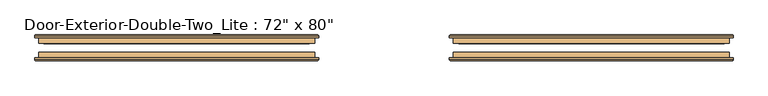
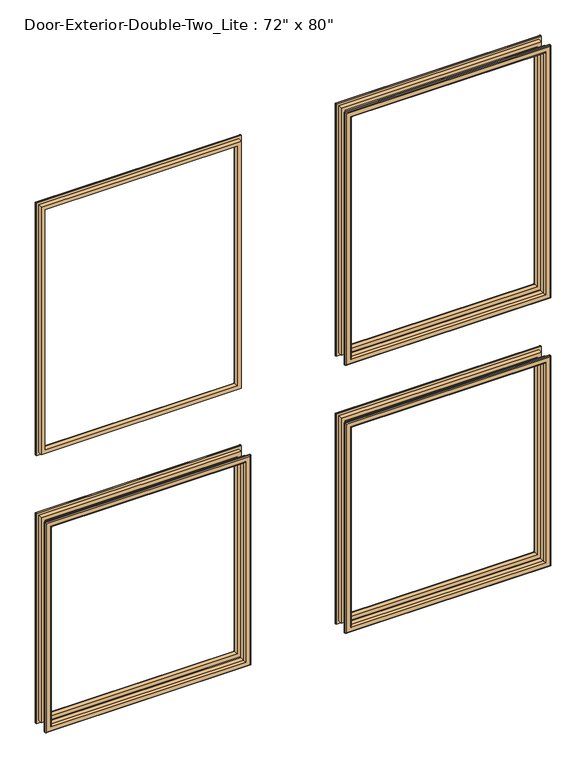
"""IFC4 building model written with IfcOpenShell, lengths in millimetres: door geometry."""

from ifc_helpers import new_model, si_unit, frame, origin, place, context, project, spatial, ellipse_curve, source, transform, mapped, element, save
from ifc_brep_helpers import plane_surface, cylinder_surface, advanced_brep


def door_4556e5f4(model_context):
    return source(origin(), model_context, "Body", "AdvancedBrep", [
        advanced_brep(
        [(-762.0, 66.675, 914.4), (-762.0, 79.375, 914.4), (-762.0, 79.375, 254.0), (-762.0, 66.675, 254.0), (-750.0, 80.375, 902.4), (-750.0, 66.675, 902.4), (-750.0, 66.675, 266.0), (-750.0, 80.375, 266.0), (-755.0, 85.375, 907.4), (-755.0, 85.375, 261.0), (-770.0, 83.375, 922.4), (-768.0, 85.375, 920.4), (-768.0, 85.375, 248.0), (-770.0, 83.375, 246.0), (-770.0, 79.375, 922.4), (-770.0, 79.375, 246.0), (-152.4, 79.375, 254.0), (-152.4, 66.675, 254.0), (-164.4, 66.675, 266.0), (-164.4, 80.375, 266.0), (-159.4, 85.375, 261.0), (-146.4, 85.375, 248.0), (-144.4, 83.375, 246.0), (-144.4, 79.375, 246.0), (-152.4, 79.375, 914.4), (-152.4, 66.675, 914.4), (-164.4, 66.675, 902.4), (-164.4, 80.375, 902.4), (-159.4, 85.375, 907.4), (-146.4, 85.375, 920.4), (-144.4, 83.375, 922.4), (-144.4, 79.375, 922.4)],
        [
            (0, 1),
            (1, 2),
            (2, 3),
            (3, 0),
            (4, 5),
            (5, 6),
            (6, 7),
            (7, 4),
            (8, 4, ellipse_curve(frame((-755.0, 80.375, 907.4), z_axis=(-0.7071067811865475, 0.0, -0.7071067811865475), x_axis=(-0.7071067811865474, 0.0, 0.7071067811865476)), 7.0710678, 5.0)),
            (7, 9, ellipse_curve(frame((-755.0, 80.375, 261.0), z_axis=(-0.7071067811865475, 0.0, 0.7071067811865475), x_axis=(0.7071067811865474, 0.0, 0.7071067811865476)), 7.0710678, 5.0)),
            (9, 8),
            (10, 11, ellipse_curve(frame((-768.0, 83.375, 920.4), z_axis=(-0.7071067811865475, 0.0, -0.7071067811865475), x_axis=(-0.7071067811865474, 0.0, 0.7071067811865476)), 2.8284271, 2.0)),
            (11, 12),
            (12, 13, ellipse_curve(frame((-768.0, 83.375, 248.0), z_axis=(-0.7071067811865475, 0.0, 0.7071067811865475), x_axis=(0.7071067811865474, 0.0, 0.7071067811865476)), 2.8284271, 2.0)),
            (13, 10),
            (14, 10),
            (13, 15),
            (15, 14),
            (2, 16),
            (16, 17),
            (17, 3),
            (6, 18),
            (18, 19),
            (19, 7),
            (19, 20, ellipse_curve(frame((-159.4, 80.375, 261.0), z_axis=(-0.7071067811865475, 0.0, -0.7071067811865475), x_axis=(-0.7071067811865476, 0.0, 0.7071067811865474)), 7.0710678, 5.0)),
            (20, 9),
            (12, 21),
            (21, 22, ellipse_curve(frame((-146.4, 83.375, 248.0), z_axis=(-0.7071067811865475, 0.0, -0.7071067811865475), x_axis=(-0.7071067811865476, 0.0, 0.7071067811865474)), 2.8284271, 2.0)),
            (22, 13),
            (22, 23),
            (23, 15),
            (16, 24),
            (24, 25),
            (25, 17),
            (18, 26),
            (26, 27),
            (27, 19),
            (27, 28, ellipse_curve(frame((-159.4, 80.375, 907.4), z_axis=(0.7071067811865475, 0.0, -0.7071067811865475), x_axis=(-0.7071067811865474, 0.0, -0.7071067811865476)), 7.0710678, 5.0)),
            (28, 20),
            (21, 29),
            (29, 30, ellipse_curve(frame((-146.4, 83.375, 920.4), z_axis=(0.7071067811865475, 0.0, -0.7071067811865475), x_axis=(-0.7071067811865474, 0.0, -0.7071067811865476)), 2.8284271, 2.0)),
            (30, 22),
            (30, 31),
            (31, 23),
            (31, 14),
            (1, 24),
            (0, 25),
            (5, 26),
            (4, 27),
            (8, 28),
            (11, 29),
            (10, 30),
        ],
        [
            plane_surface(frame((-762.0, 79.375, 914.4), z_axis=(-1.0, 0.0, 0.0), x_axis=(0.0, 0.0, -1.0))),
            plane_surface(frame((-750.0, 66.675, 902.4), z_axis=(1.0, 0.0, 0.0), x_axis=(0.0, 0.0, -1.0))),
            cylinder_surface(frame((-755.0, 80.375, 914.4), z_axis=(0.0, 0.0, 1.0), x_axis=(-1.0, 0.0, 0.0)), 5.0),
            cylinder_surface(frame((-768.0, 83.375, 914.4), z_axis=(0.0, 0.0, 1.0), x_axis=(-1.0, 0.0, 0.0)), 2.0),
            plane_surface(frame((-770.0, 83.375, 922.4), z_axis=(-1.0, 0.0, 0.0), x_axis=(0.0, 0.0, -1.0))),
            plane_surface(frame((-762.0, 79.375, 254.0), z_axis=(0.0, 0.0, -1.0), x_axis=(1.0, 0.0, 0.0))),
            plane_surface(frame((-750.0, 66.675, 266.0), z_axis=(0.0, 0.0, 1.0), x_axis=(1.0, 0.0, 0.0))),
            cylinder_surface(frame((-762.0, 80.375, 261.0), z_axis=(-1.0, 0.0, 0.0), x_axis=(0.0, 0.0, -1.0)), 5.0),
            cylinder_surface(frame((-762.0, 83.375, 248.0), z_axis=(-1.0, 0.0, 0.0), x_axis=(0.0, 0.0, -1.0)), 2.0),
            plane_surface(frame((-770.0, 83.375, 246.0), z_axis=(0.0, 0.0, -1.0), x_axis=(1.0, 0.0, 0.0))),
            plane_surface(frame((-152.4, 79.375, 254.0), z_axis=(1.0, 0.0, 0.0), x_axis=(0.0, 0.0, 1.0))),
            plane_surface(frame((-164.4, 66.675, 266.0), z_axis=(-1.0, 0.0, 0.0), x_axis=(0.0, 0.0, 1.0))),
            cylinder_surface(frame((-159.4, 80.375, 254.0), z_axis=(0.0, 0.0, -1.0), x_axis=(1.0, 0.0, 0.0)), 5.0),
            cylinder_surface(frame((-146.4, 83.375, 254.0), z_axis=(0.0, 0.0, -1.0), x_axis=(1.0, 0.0, 0.0)), 2.0),
            plane_surface(frame((-144.4, 83.375, 246.0), z_axis=(1.0, 0.0, 0.0), x_axis=(0.0, 0.0, 1.0))),
            plane_surface(frame((-144.4, 79.375, 922.4), z_axis=(0.0, -1.0, 0.0), x_axis=(-1.0, 0.0, 0.0))),
            plane_surface(frame((-152.4, 79.375, 914.4), z_axis=(0.0, 0.0, 1.0), x_axis=(-1.0, 0.0, 0.0))),
            plane_surface(frame((-152.4, 66.675, 914.4), z_axis=(0.0, -1.0, 0.0), x_axis=(-1.0, 0.0, 0.0))),
            plane_surface(frame((-164.4, 66.675, 902.4), z_axis=(0.0, 0.0, -1.0), x_axis=(-1.0, 0.0, 0.0))),
            cylinder_surface(frame((-152.4, 80.375, 907.4), z_axis=(1.0, 0.0, 0.0), x_axis=(0.0, 0.0, 1.0)), 5.0),
            plane_surface(frame((-159.4, 85.375, 907.4), z_axis=(0.0, 1.0, 0.0), x_axis=(-1.0, 0.0, 0.0))),
            cylinder_surface(frame((-152.4, 83.375, 920.4), z_axis=(1.0, 0.0, 0.0), x_axis=(0.0, 0.0, 1.0)), 2.0),
            plane_surface(frame((-144.4, 83.375, 922.4), z_axis=(0.0, 0.0, 1.0), x_axis=(-1.0, 0.0, 0.0))),
        ],
        [
            (0, [[1, 2, 3, 4]]),
            (1, [[5, 6, 7, 8]]),
            (2, [[9, -8, 10, 11]]),
            (3, [[12, 13, 14, 15]]),
            (4, [[16, -15, 17, 18]]),
            (5, [[-3, 19, 20, 21]]),
            (6, [[-7, 22, 23, 24]]),
            (7, [[-10, -24, 25, 26]]),
            (8, [[-14, 27, 28, 29]]),
            (9, [[-17, -29, 30, 31]]),
            (10, [[-20, 32, 33, 34]]),
            (11, [[-23, 35, 36, 37]]),
            (12, [[-25, -37, 38, 39]]),
            (13, [[-28, 40, 41, 42]]),
            (14, [[-30, -42, 43, 44]]),
            (15, [[-31, -44, 45, -18], [46, -32, -19, -2]]),
            (16, [[-33, -46, -1, 47]]),
            (17, [[-21, -34, -47, -4], [48, -35, -22, -6]]),
            (18, [[-36, -48, -5, 49]]),
            (19, [[-38, -49, -9, 50]]),
            (20, [[51, -40, -27, -13], [-26, -39, -50, -11]]),
            (21, [[-41, -51, -12, 52]]),
            (22, [[-43, -52, -16, -45]]),
        ],
    ),
        advanced_brep(
        [(152.4, 66.675, 914.4), (152.4, 79.375, 914.4), (152.4, 79.375, 254.0), (152.4, 66.675, 254.0), (164.4, 80.375, 902.4), (164.4, 66.675, 902.4), (164.4, 66.675, 266.0), (164.4, 80.375, 266.0), (159.4, 85.375, 907.4), (159.4, 85.375, 261.0), (144.4, 83.375, 922.4), (146.4, 85.375, 920.4), (146.4, 85.375, 248.0), (144.4, 83.375, 246.0), (144.4, 79.375, 922.4), (144.4, 79.375, 246.0), (762.0, 79.375, 254.0), (762.0, 66.675, 254.0), (750.0, 66.675, 266.0), (750.0, 80.375, 266.0), (755.0, 85.375, 261.0), (768.0, 85.375, 248.0), (770.0, 83.375, 246.0), (770.0, 79.375, 246.0), (762.0, 79.375, 914.4), (762.0, 66.675, 914.4), (750.0, 66.675, 902.4), (750.0, 80.375, 902.4), (755.0, 85.375, 907.4), (768.0, 85.375, 920.4), (770.0, 83.375, 922.4), (770.0, 79.375, 922.4)],
        [
            (0, 1),
            (1, 2),
            (2, 3),
            (3, 0),
            (4, 5),
            (5, 6),
            (6, 7),
            (7, 4),
            (8, 4, ellipse_curve(frame((159.4, 80.375, 907.4), z_axis=(-0.7071067811865475, 0.0, -0.7071067811865475), x_axis=(-0.7071067811865474, 0.0, 0.7071067811865476)), 7.0710678, 5.0)),
            (7, 9, ellipse_curve(frame((159.4, 80.375, 261.0), z_axis=(-0.7071067811865475, 0.0, 0.7071067811865475), x_axis=(0.7071067811865474, 0.0, 0.7071067811865476)), 7.0710678, 5.0)),
            (9, 8),
            (10, 11, ellipse_curve(frame((146.4, 83.375, 920.4), z_axis=(-0.7071067811865475, 0.0, -0.7071067811865475), x_axis=(-0.7071067811865474, 0.0, 0.7071067811865476)), 2.8284271, 2.0)),
            (11, 12),
            (12, 13, ellipse_curve(frame((146.4, 83.375, 248.0), z_axis=(-0.7071067811865475, 0.0, 0.7071067811865475), x_axis=(0.7071067811865474, 0.0, 0.7071067811865476)), 2.8284271, 2.0)),
            (13, 10),
            (14, 10),
            (13, 15),
            (15, 14),
            (2, 16),
            (16, 17),
            (17, 3),
            (6, 18),
            (18, 19),
            (19, 7),
            (19, 20, ellipse_curve(frame((755.0, 80.375, 261.0), z_axis=(-0.7071067811865475, 0.0, -0.7071067811865475), x_axis=(-0.7071067811865476, 0.0, 0.7071067811865474)), 7.0710678, 5.0)),
            (20, 9),
            (12, 21),
            (21, 22, ellipse_curve(frame((768.0, 83.375, 248.0), z_axis=(-0.7071067811865475, 0.0, -0.7071067811865475), x_axis=(-0.7071067811865476, 0.0, 0.7071067811865474)), 2.8284271, 2.0)),
            (22, 13),
            (22, 23),
            (23, 15),
            (16, 24),
            (24, 25),
            (25, 17),
            (18, 26),
            (26, 27),
            (27, 19),
            (27, 28, ellipse_curve(frame((755.0, 80.375, 907.4), z_axis=(0.7071067811865475, 0.0, -0.7071067811865475), x_axis=(-0.7071067811865474, 0.0, -0.7071067811865476)), 7.0710678, 5.0)),
            (28, 20),
            (21, 29),
            (29, 30, ellipse_curve(frame((768.0, 83.375, 920.4), z_axis=(0.7071067811865475, 0.0, -0.7071067811865475), x_axis=(-0.7071067811865474, 0.0, -0.7071067811865476)), 2.8284271, 2.0)),
            (30, 22),
            (30, 31),
            (31, 23),
            (31, 14),
            (1, 24),
            (0, 25),
            (5, 26),
            (4, 27),
            (8, 28),
            (11, 29),
            (10, 30),
        ],
        [
            plane_surface(frame((152.4, 79.375, 914.4), z_axis=(-1.0, 0.0, 0.0), x_axis=(0.0, 0.0, -1.0))),
            plane_surface(frame((164.4, 66.675, 902.4), z_axis=(1.0, 0.0, 0.0), x_axis=(0.0, 0.0, -1.0))),
            cylinder_surface(frame((159.4, 80.375, 914.4), z_axis=(0.0, 0.0, 1.0), x_axis=(-1.0, 0.0, 0.0)), 5.0),
            cylinder_surface(frame((146.4, 83.375, 914.4), z_axis=(0.0, 0.0, 1.0), x_axis=(-1.0, 0.0, 0.0)), 2.0),
            plane_surface(frame((144.4, 83.375, 922.4), z_axis=(-1.0, 0.0, 0.0), x_axis=(0.0, 0.0, -1.0))),
            plane_surface(frame((152.4, 79.375, 254.0), z_axis=(0.0, 0.0, -1.0), x_axis=(1.0, 0.0, 0.0))),
            plane_surface(frame((164.4, 66.675, 266.0), z_axis=(0.0, 0.0, 1.0), x_axis=(1.0, 0.0, 0.0))),
            cylinder_surface(frame((152.4, 80.375, 261.0), z_axis=(-1.0, 0.0, 0.0), x_axis=(0.0, 0.0, -1.0)), 5.0),
            cylinder_surface(frame((152.4, 83.375, 248.0), z_axis=(-1.0, 0.0, 0.0), x_axis=(0.0, 0.0, -1.0)), 2.0),
            plane_surface(frame((144.4, 83.375, 246.0), z_axis=(0.0, 0.0, -1.0), x_axis=(1.0, 0.0, 0.0))),
            plane_surface(frame((762.0, 79.375, 254.0), z_axis=(1.0, 0.0, 0.0), x_axis=(0.0, 0.0, 1.0))),
            plane_surface(frame((750.0, 66.675, 266.0), z_axis=(-1.0, 0.0, 0.0), x_axis=(0.0, 0.0, 1.0))),
            cylinder_surface(frame((755.0, 80.375, 254.0), z_axis=(0.0, 0.0, -1.0), x_axis=(1.0, 0.0, 0.0)), 5.0),
            cylinder_surface(frame((768.0, 83.375, 254.0), z_axis=(0.0, 0.0, -1.0), x_axis=(1.0, 0.0, 0.0)), 2.0),
            plane_surface(frame((770.0, 83.375, 246.0), z_axis=(1.0, 0.0, 0.0), x_axis=(0.0, 0.0, 1.0))),
            plane_surface(frame((770.0, 79.375, 922.4), z_axis=(0.0, -1.0, 0.0), x_axis=(-1.0, 0.0, 0.0))),
            plane_surface(frame((762.0, 79.375, 914.4), z_axis=(0.0, 0.0, 1.0), x_axis=(-1.0, 0.0, 0.0))),
            plane_surface(frame((762.0, 66.675, 914.4), z_axis=(0.0, -1.0, 0.0), x_axis=(-1.0, 0.0, 0.0))),
            plane_surface(frame((750.0, 66.675, 902.4), z_axis=(0.0, 0.0, -1.0), x_axis=(-1.0, 0.0, 0.0))),
            cylinder_surface(frame((762.0, 80.375, 907.4), z_axis=(1.0, 0.0, 0.0), x_axis=(0.0, 0.0, 1.0)), 5.0),
            plane_surface(frame((755.0, 85.375, 907.4), z_axis=(0.0, 1.0, 0.0), x_axis=(-1.0, 0.0, 0.0))),
            cylinder_surface(frame((762.0, 83.375, 920.4), z_axis=(1.0, 0.0, 0.0), x_axis=(0.0, 0.0, 1.0)), 2.0),
            plane_surface(frame((770.0, 83.375, 922.4), z_axis=(0.0, 0.0, 1.0), x_axis=(-1.0, 0.0, 0.0))),
        ],
        [
            (0, [[1, 2, 3, 4]]),
            (1, [[5, 6, 7, 8]]),
            (2, [[9, -8, 10, 11]]),
            (3, [[12, 13, 14, 15]]),
            (4, [[16, -15, 17, 18]]),
            (5, [[-3, 19, 20, 21]]),
            (6, [[-7, 22, 23, 24]]),
            (7, [[-10, -24, 25, 26]]),
            (8, [[-14, 27, 28, 29]]),
            (9, [[-17, -29, 30, 31]]),
            (10, [[-20, 32, 33, 34]]),
            (11, [[-23, 35, 36, 37]]),
            (12, [[-25, -37, 38, 39]]),
            (13, [[-28, 40, 41, 42]]),
            (14, [[-30, -42, 43, 44]]),
            (15, [[-31, -44, 45, -18], [46, -32, -19, -2]]),
            (16, [[-33, -46, -1, 47]]),
            (17, [[-21, -34, -47, -4], [48, -35, -22, -6]]),
            (18, [[-36, -48, -5, 49]]),
            (19, [[-38, -49, -9, 50]]),
            (20, [[51, -40, -27, -13], [-26, -39, -50, -11]]),
            (21, [[-41, -51, -12, 52]]),
            (22, [[-43, -52, -16, -45]]),
        ],
    ),
        advanced_brep(
        [(152.4, 66.675, 1914.525), (152.4, 79.375, 1914.525), (152.4, 79.375, 1117.6), (152.4, 66.675, 1117.6), (164.4, 80.375, 1902.525), (164.4, 66.675, 1902.525), (164.4, 66.675, 1129.6), (164.4, 80.375, 1129.6), (159.4, 85.375, 1907.525), (159.4, 85.375, 1124.6), (144.4, 83.375, 1922.525), (146.4, 85.375, 1920.525), (146.4, 85.375, 1111.6), (144.4, 83.375, 1109.6), (144.4, 79.375, 1922.525), (144.4, 79.375, 1109.6), (762.0, 79.375, 1117.6), (762.0, 66.675, 1117.6), (750.0, 66.675, 1129.6), (750.0, 80.375, 1129.6), (755.0, 85.375, 1124.6), (768.0, 85.375, 1111.6), (770.0, 83.375, 1109.6), (770.0, 79.375, 1109.6), (762.0, 79.375, 1914.525), (762.0, 66.675, 1914.525), (750.0, 66.675, 1902.525), (750.0, 80.375, 1902.525), (755.0, 85.375, 1907.525), (768.0, 85.375, 1920.525), (770.0, 83.375, 1922.525), (770.0, 79.375, 1922.525)],
        [
            (0, 1),
            (1, 2),
            (2, 3),
            (3, 0),
            (4, 5),
            (5, 6),
            (6, 7),
            (7, 4),
            (8, 4, ellipse_curve(frame((159.4, 80.375, 1907.525), z_axis=(-0.7071067811865475, 0.0, -0.7071067811865475), x_axis=(-0.7071067811865474, 0.0, 0.7071067811865476)), 7.0710678, 5.0)),
            (7, 9, ellipse_curve(frame((159.4, 80.375, 1124.6), z_axis=(-0.7071067811865475, 0.0, 0.7071067811865475), x_axis=(0.7071067811865474, 0.0, 0.7071067811865476)), 7.0710678, 5.0)),
            (9, 8),
            (10, 11, ellipse_curve(frame((146.4, 83.375, 1920.525), z_axis=(-0.7071067811865475, 0.0, -0.7071067811865475), x_axis=(-0.7071067811865474, 0.0, 0.7071067811865476)), 2.8284271, 2.0)),
            (11, 12),
            (12, 13, ellipse_curve(frame((146.4, 83.375, 1111.6), z_axis=(-0.7071067811865475, 0.0, 0.7071067811865475), x_axis=(0.7071067811865474, 0.0, 0.7071067811865476)), 2.8284271, 2.0)),
            (13, 10),
            (14, 10),
            (13, 15),
            (15, 14),
            (2, 16),
            (16, 17),
            (17, 3),
            (6, 18),
            (18, 19),
            (19, 7),
            (19, 20, ellipse_curve(frame((755.0, 80.375, 1124.6), z_axis=(-0.7071067811865475, 0.0, -0.7071067811865475), x_axis=(-0.7071067811865476, 0.0, 0.7071067811865474)), 7.0710678, 5.0)),
            (20, 9),
            (12, 21),
            (21, 22, ellipse_curve(frame((768.0, 83.375, 1111.6), z_axis=(-0.7071067811865475, 0.0, -0.7071067811865475), x_axis=(-0.7071067811865476, 0.0, 0.7071067811865474)), 2.8284271, 2.0)),
            (22, 13),
            (22, 23),
            (23, 15),
            (16, 24),
            (24, 25),
            (25, 17),
            (18, 26),
            (26, 27),
            (27, 19),
            (27, 28, ellipse_curve(frame((755.0, 80.375, 1907.525), z_axis=(0.7071067811865475, 0.0, -0.7071067811865475), x_axis=(-0.7071067811865474, 0.0, -0.7071067811865476)), 7.0710678, 5.0)),
            (28, 20),
            (21, 29),
            (29, 30, ellipse_curve(frame((768.0, 83.375, 1920.525), z_axis=(0.7071067811865475, 0.0, -0.7071067811865475), x_axis=(-0.7071067811865474, 0.0, -0.7071067811865476)), 2.8284271, 2.0)),
            (30, 22),
            (30, 31),
            (31, 23),
            (31, 14),
            (1, 24),
            (0, 25),
            (5, 26),
            (4, 27),
            (8, 28),
            (11, 29),
            (10, 30),
        ],
        [
            plane_surface(frame((152.4, 79.375, 1914.525), z_axis=(-1.0, 0.0, 0.0), x_axis=(0.0, 0.0, -1.0))),
            plane_surface(frame((164.4, 66.675, 1902.525), z_axis=(1.0, 0.0, 0.0), x_axis=(0.0, 0.0, -1.0))),
            cylinder_surface(frame((159.4, 80.375, 1914.525), z_axis=(0.0, 0.0, 1.0), x_axis=(-1.0, 0.0, 0.0)), 5.0),
            cylinder_surface(frame((146.4, 83.375, 1914.525), z_axis=(0.0, 0.0, 1.0), x_axis=(-1.0, 0.0, 0.0)), 2.0),
            plane_surface(frame((144.4, 83.375, 1922.525), z_axis=(-1.0, 0.0, 0.0), x_axis=(0.0, 0.0, -1.0))),
            plane_surface(frame((152.4, 79.375, 1117.6), z_axis=(0.0, 0.0, -1.0), x_axis=(1.0, 0.0, 0.0))),
            plane_surface(frame((164.4, 66.675, 1129.6), z_axis=(0.0, 0.0, 1.0), x_axis=(1.0, 0.0, 0.0))),
            cylinder_surface(frame((152.4, 80.375, 1124.6), z_axis=(-1.0, 0.0, 0.0), x_axis=(0.0, 0.0, -1.0)), 5.0),
            cylinder_surface(frame((152.4, 83.375, 1111.6), z_axis=(-1.0, 0.0, 0.0), x_axis=(0.0, 0.0, -1.0)), 2.0),
            plane_surface(frame((144.4, 83.375, 1109.6), z_axis=(0.0, 0.0, -1.0), x_axis=(1.0, 0.0, 0.0))),
            plane_surface(frame((762.0, 79.375, 1117.6), z_axis=(1.0, 0.0, 0.0), x_axis=(0.0, 0.0, 1.0))),
            plane_surface(frame((750.0, 66.675, 1129.6), z_axis=(-1.0, 0.0, 0.0), x_axis=(0.0, 0.0, 1.0))),
            cylinder_surface(frame((755.0, 80.375, 1117.6), z_axis=(0.0, 0.0, -1.0), x_axis=(1.0, 0.0, 0.0)), 5.0),
            cylinder_surface(frame((768.0, 83.375, 1117.6), z_axis=(0.0, 0.0, -1.0), x_axis=(1.0, 0.0, 0.0)), 2.0),
            plane_surface(frame((770.0, 83.375, 1109.6), z_axis=(1.0, 0.0, 0.0), x_axis=(0.0, 0.0, 1.0))),
            plane_surface(frame((770.0, 79.375, 1922.525), z_axis=(0.0, -1.0, 0.0), x_axis=(-1.0, 0.0, 0.0))),
            plane_surface(frame((762.0, 79.375, 1914.525), z_axis=(0.0, 0.0, 1.0), x_axis=(-1.0, 0.0, 0.0))),
            plane_surface(frame((762.0, 66.675, 1914.525), z_axis=(0.0, -1.0, 0.0), x_axis=(-1.0, 0.0, 0.0))),
            plane_surface(frame((750.0, 66.675, 1902.525), z_axis=(0.0, 0.0, -1.0), x_axis=(-1.0, 0.0, 0.0))),
            cylinder_surface(frame((762.0, 80.375, 1907.525), z_axis=(1.0, 0.0, 0.0), x_axis=(0.0, 0.0, 1.0)), 5.0),
            plane_surface(frame((755.0, 85.375, 1907.525), z_axis=(0.0, 1.0, 0.0), x_axis=(-1.0, 0.0, 0.0))),
            cylinder_surface(frame((762.0, 83.375, 1920.525), z_axis=(1.0, 0.0, 0.0), x_axis=(0.0, 0.0, 1.0)), 2.0),
            plane_surface(frame((770.0, 83.375, 1922.525), z_axis=(0.0, 0.0, 1.0), x_axis=(-1.0, 0.0, 0.0))),
        ],
        [
            (0, [[1, 2, 3, 4]]),
            (1, [[5, 6, 7, 8]]),
            (2, [[9, -8, 10, 11]]),
            (3, [[12, 13, 14, 15]]),
            (4, [[16, -15, 17, 18]]),
            (5, [[-3, 19, 20, 21]]),
            (6, [[-7, 22, 23, 24]]),
            (7, [[-10, -24, 25, 26]]),
            (8, [[-14, 27, 28, 29]]),
            (9, [[-17, -29, 30, 31]]),
            (10, [[-20, 32, 33, 34]]),
            (11, [[-23, 35, 36, 37]]),
            (12, [[-25, -37, 38, 39]]),
            (13, [[-28, 40, 41, 42]]),
            (14, [[-30, -42, 43, 44]]),
            (15, [[-31, -44, 45, -18], [46, -32, -19, -2]]),
            (16, [[-33, -46, -1, 47]]),
            (17, [[-21, -34, -47, -4], [48, -35, -22, -6]]),
            (18, [[-36, -48, -5, 49]]),
            (19, [[-38, -49, -9, 50]]),
            (20, [[51, -40, -27, -13], [-26, -39, -50, -11]]),
            (21, [[-41, -51, -12, 52]]),
            (22, [[-43, -52, -16, -45]]),
        ],
    ),
        advanced_brep(
        [(-762.0, 66.675, 1914.525), (-762.0, 79.375, 1914.525), (-762.0, 79.375, 1117.6), (-762.0, 66.675, 1117.6), (-750.0, 80.375, 1902.525), (-750.0, 66.675, 1902.525), (-750.0, 66.675, 1129.6), (-750.0, 80.375, 1129.6), (-755.0, 85.375, 1907.525), (-755.0, 85.375, 1124.6), (-770.0, 83.375, 1922.525), (-768.0, 85.375, 1920.525), (-768.0, 85.375, 1111.6), (-770.0, 83.375, 1109.6), (-770.0, 79.375, 1922.525), (-770.0, 79.375, 1109.6), (-152.4, 79.375, 1117.6), (-152.4, 66.675, 1117.6), (-164.4, 66.675, 1129.6), (-164.4, 80.375, 1129.6), (-159.4, 85.375, 1124.6), (-146.4, 85.375, 1111.6), (-144.4, 83.375, 1109.6), (-144.4, 79.375, 1109.6), (-152.4, 79.375, 1914.525), (-152.4, 66.675, 1914.525), (-164.4, 66.675, 1902.525), (-164.4, 80.375, 1902.525), (-159.4, 85.375, 1907.525), (-146.4, 85.375, 1920.525), (-144.4, 83.375, 1922.525), (-144.4, 79.375, 1922.525)],
        [
            (0, 1),
            (1, 2),
            (2, 3),
            (3, 0),
            (4, 5),
            (5, 6),
            (6, 7),
            (7, 4),
            (8, 4, ellipse_curve(frame((-755.0, 80.375, 1907.525), z_axis=(-0.7071067811865475, 0.0, -0.7071067811865475), x_axis=(-0.7071067811865474, 0.0, 0.7071067811865476)), 7.0710678, 5.0)),
            (7, 9, ellipse_curve(frame((-755.0, 80.375, 1124.6), z_axis=(-0.7071067811865475, 0.0, 0.7071067811865475), x_axis=(0.7071067811865474, 0.0, 0.7071067811865476)), 7.0710678, 5.0)),
            (9, 8),
            (10, 11, ellipse_curve(frame((-768.0, 83.375, 1920.525), z_axis=(-0.7071067811865475, 0.0, -0.7071067811865475), x_axis=(-0.7071067811865474, 0.0, 0.7071067811865476)), 2.8284271, 2.0)),
            (11, 12),
            (12, 13, ellipse_curve(frame((-768.0, 83.375, 1111.6), z_axis=(-0.7071067811865475, 0.0, 0.7071067811865475), x_axis=(0.7071067811865474, 0.0, 0.7071067811865476)), 2.8284271, 2.0)),
            (13, 10),
            (14, 10),
            (13, 15),
            (15, 14),
            (2, 16),
            (16, 17),
            (17, 3),
            (6, 18),
            (18, 19),
            (19, 7),
            (19, 20, ellipse_curve(frame((-159.4, 80.375, 1124.6), z_axis=(-0.7071067811865475, 0.0, -0.7071067811865475), x_axis=(-0.7071067811865476, 0.0, 0.7071067811865474)), 7.0710678, 5.0)),
            (20, 9),
            (12, 21),
            (21, 22, ellipse_curve(frame((-146.4, 83.375, 1111.6), z_axis=(-0.7071067811865475, 0.0, -0.7071067811865475), x_axis=(-0.7071067811865476, 0.0, 0.7071067811865474)), 2.8284271, 2.0)),
            (22, 13),
            (22, 23),
            (23, 15),
            (16, 24),
            (24, 25),
            (25, 17),
            (18, 26),
            (26, 27),
            (27, 19),
            (27, 28, ellipse_curve(frame((-159.4, 80.375, 1907.525), z_axis=(0.7071067811865475, 0.0, -0.7071067811865475), x_axis=(-0.7071067811865474, 0.0, -0.7071067811865476)), 7.0710678, 5.0)),
            (28, 20),
            (21, 29),
            (29, 30, ellipse_curve(frame((-146.4, 83.375, 1920.525), z_axis=(0.7071067811865475, 0.0, -0.7071067811865475), x_axis=(-0.7071067811865474, 0.0, -0.7071067811865476)), 2.8284271, 2.0)),
            (30, 22),
            (30, 31),
            (31, 23),
            (31, 14),
            (1, 24),
            (0, 25),
            (5, 26),
            (4, 27),
            (8, 28),
            (11, 29),
            (10, 30),
        ],
        [
            plane_surface(frame((-762.0, 79.375, 1914.525), z_axis=(-1.0, 0.0, 0.0), x_axis=(0.0, 0.0, -1.0))),
            plane_surface(frame((-750.0, 66.675, 1902.525), z_axis=(1.0, 0.0, 0.0), x_axis=(0.0, 0.0, -1.0))),
            cylinder_surface(frame((-755.0, 80.375, 1914.525), z_axis=(0.0, 0.0, 1.0), x_axis=(-1.0, 0.0, 0.0)), 5.0),
            cylinder_surface(frame((-768.0, 83.375, 1914.525), z_axis=(0.0, 0.0, 1.0), x_axis=(-1.0, 0.0, 0.0)), 2.0),
            plane_surface(frame((-770.0, 83.375, 1922.525), z_axis=(-1.0, 0.0, 0.0), x_axis=(0.0, 0.0, -1.0))),
            plane_surface(frame((-762.0, 79.375, 1117.6), z_axis=(0.0, 0.0, -1.0), x_axis=(1.0, 0.0, 0.0))),
            plane_surface(frame((-750.0, 66.675, 1129.6), z_axis=(0.0, 0.0, 1.0), x_axis=(1.0, 0.0, 0.0))),
            cylinder_surface(frame((-762.0, 80.375, 1124.6), z_axis=(-1.0, 0.0, 0.0), x_axis=(0.0, 0.0, -1.0)), 5.0),
            cylinder_surface(frame((-762.0, 83.375, 1111.6), z_axis=(-1.0, 0.0, 0.0), x_axis=(0.0, 0.0, -1.0)), 2.0),
            plane_surface(frame((-770.0, 83.375, 1109.6), z_axis=(0.0, 0.0, -1.0), x_axis=(1.0, 0.0, 0.0))),
            plane_surface(frame((-152.4, 79.375, 1117.6), z_axis=(1.0, 0.0, 0.0), x_axis=(0.0, 0.0, 1.0))),
            plane_surface(frame((-164.4, 66.675, 1129.6), z_axis=(-1.0, 0.0, 0.0), x_axis=(0.0, 0.0, 1.0))),
            cylinder_surface(frame((-159.4, 80.375, 1117.6), z_axis=(0.0, 0.0, -1.0), x_axis=(1.0, 0.0, 0.0)), 5.0),
            cylinder_surface(frame((-146.4, 83.375, 1117.6), z_axis=(0.0, 0.0, -1.0), x_axis=(1.0, 0.0, 0.0)), 2.0),
            plane_surface(frame((-144.4, 83.375, 1109.6), z_axis=(1.0, 0.0, 0.0), x_axis=(0.0, 0.0, 1.0))),
            plane_surface(frame((-144.4, 79.375, 1922.525), z_axis=(0.0, -1.0, 0.0), x_axis=(-1.0, 0.0, 0.0))),
            plane_surface(frame((-152.4, 79.375, 1914.525), z_axis=(0.0, 0.0, 1.0), x_axis=(-1.0, 0.0, 0.0))),
            plane_surface(frame((-152.4, 66.675, 1914.525), z_axis=(0.0, -1.0, 0.0), x_axis=(-1.0, 0.0, 0.0))),
            plane_surface(frame((-164.4, 66.675, 1902.525), z_axis=(0.0, 0.0, -1.0), x_axis=(-1.0, 0.0, 0.0))),
            cylinder_surface(frame((-152.4, 80.375, 1907.525), z_axis=(1.0, 0.0, 0.0), x_axis=(0.0, 0.0, 1.0)), 5.0),
            plane_surface(frame((-159.4, 85.375, 1907.525), z_axis=(0.0, 1.0, 0.0), x_axis=(-1.0, 0.0, 0.0))),
            cylinder_surface(frame((-152.4, 83.375, 1920.525), z_axis=(1.0, 0.0, 0.0), x_axis=(0.0, 0.0, 1.0)), 2.0),
            plane_surface(frame((-144.4, 83.375, 1922.525), z_axis=(0.0, 0.0, 1.0), x_axis=(-1.0, 0.0, 0.0))),
        ],
        [
            (0, [[1, 2, 3, 4]]),
            (1, [[5, 6, 7, 8]]),
            (2, [[9, -8, 10, 11]]),
            (3, [[12, 13, 14, 15]]),
            (4, [[16, -15, 17, 18]]),
            (5, [[-3, 19, 20, 21]]),
            (6, [[-7, 22, 23, 24]]),
            (7, [[-10, -24, 25, 26]]),
            (8, [[-14, 27, 28, 29]]),
            (9, [[-17, -29, 30, 31]]),
            (10, [[-20, 32, 33, 34]]),
            (11, [[-23, 35, 36, 37]]),
            (12, [[-25, -37, 38, 39]]),
            (13, [[-28, 40, 41, 42]]),
            (14, [[-30, -42, 43, 44]]),
            (15, [[-31, -44, 45, -18], [46, -32, -19, -2]]),
            (16, [[-33, -46, -1, 47]]),
            (17, [[-21, -34, -47, -4], [48, -35, -22, -6]]),
            (18, [[-36, -48, -5, 49]]),
            (19, [[-38, -49, -9, 50]]),
            (20, [[51, -40, -27, -13], [-26, -39, -50, -11]]),
            (21, [[-41, -51, -12, 52]]),
            (22, [[-43, -52, -16, -45]]),
        ],
    ),
        advanced_brep(
        [(-762.0, 47.625, 254.0), (-762.0, 34.925, 254.0), (-762.0, 34.925, 914.4), (-762.0, 47.625, 914.4), (-750.0, 33.925, 266.0), (-750.0, 47.625, 266.0), (-750.0, 47.625, 902.4), (-750.0, 33.925, 902.4), (-755.0, 28.925, 261.0), (-755.0, 28.925, 907.4), (-770.0, 30.925, 246.0), (-768.0, 28.925, 248.0), (-768.0, 28.925, 920.4), (-770.0, 30.925, 922.4), (-770.0, 34.925, 246.0), (-770.0, 34.925, 922.4), (-152.4, 34.925, 914.4), (-152.4, 47.625, 914.4), (-164.4, 47.625, 902.4), (-164.4, 33.925, 902.4), (-159.4, 28.925, 907.4), (-146.4, 28.925, 920.4), (-144.4, 30.925, 922.4), (-144.4, 34.925, 922.4), (-152.4, 34.925, 254.0), (-152.4, 47.625, 254.0), (-164.4, 47.625, 266.0), (-164.4, 33.925, 266.0), (-159.4, 28.925, 261.0), (-146.4, 28.925, 248.0), (-144.4, 30.925, 246.0), (-144.4, 34.925, 246.0)],
        [
            (0, 1),
            (1, 2),
            (2, 3),
            (3, 0),
            (4, 5),
            (5, 6),
            (6, 7),
            (7, 4),
            (8, 4, ellipse_curve(frame((-755.0, 33.925, 261.0), z_axis=(-0.7071067811865475, 0.0, 0.7071067811865475), x_axis=(-0.7071067811865474, 0.0, -0.7071067811865476)), 7.0710678, 5.0)),
            (7, 9, ellipse_curve(frame((-755.0, 33.925, 907.4), z_axis=(-0.7071067811865475, 0.0, -0.7071067811865475), x_axis=(0.7071067811865474, 0.0, -0.7071067811865476)), 7.0710678, 5.0)),
            (9, 8),
            (10, 11, ellipse_curve(frame((-768.0, 30.925, 248.0), z_axis=(-0.7071067811865475, 0.0, 0.7071067811865475), x_axis=(-0.7071067811865474, 0.0, -0.7071067811865476)), 2.8284271, 2.0)),
            (11, 12),
            (12, 13, ellipse_curve(frame((-768.0, 30.925, 920.4), z_axis=(-0.7071067811865475, 0.0, -0.7071067811865475), x_axis=(0.7071067811865474, 0.0, -0.7071067811865476)), 2.8284271, 2.0)),
            (13, 10),
            (14, 10),
            (13, 15),
            (15, 14),
            (2, 16),
            (16, 17),
            (17, 3),
            (6, 18),
            (18, 19),
            (19, 7),
            (19, 20, ellipse_curve(frame((-159.4, 33.925, 907.4), z_axis=(-0.7071067811865475, 0.0, 0.7071067811865475), x_axis=(-0.7071067811865476, 0.0, -0.7071067811865474)), 7.0710678, 5.0)),
            (20, 9),
            (12, 21),
            (21, 22, ellipse_curve(frame((-146.4, 30.925, 920.4), z_axis=(-0.7071067811865475, 0.0, 0.7071067811865475), x_axis=(-0.7071067811865476, 0.0, -0.7071067811865474)), 2.8284271, 2.0)),
            (22, 13),
            (22, 23),
            (23, 15),
            (16, 24),
            (24, 25),
            (25, 17),
            (18, 26),
            (26, 27),
            (27, 19),
            (27, 28, ellipse_curve(frame((-159.4, 33.925, 261.0), z_axis=(0.7071067811865475, 0.0, 0.7071067811865475), x_axis=(-0.7071067811865474, 0.0, 0.7071067811865476)), 7.0710678, 5.0)),
            (28, 20),
            (21, 29),
            (29, 30, ellipse_curve(frame((-146.4, 30.925, 248.0), z_axis=(0.7071067811865475, 0.0, 0.7071067811865475), x_axis=(-0.7071067811865474, 0.0, 0.7071067811865476)), 2.8284271, 2.0)),
            (30, 22),
            (30, 31),
            (31, 23),
            (31, 14),
            (1, 24),
            (0, 25),
            (5, 26),
            (4, 27),
            (8, 28),
            (11, 29),
            (10, 30),
        ],
        [
            plane_surface(frame((-762.0, 34.925, 254.0), z_axis=(-1.0, 0.0, 0.0), x_axis=(0.0, 0.0, 1.0))),
            plane_surface(frame((-750.0, 47.625, 266.0), z_axis=(1.0, 0.0, 0.0), x_axis=(0.0, 0.0, 1.0))),
            cylinder_surface(frame((-755.0, 33.925, 254.0), z_axis=(0.0, 0.0, -1.0), x_axis=(-1.0, 0.0, 0.0)), 5.0),
            cylinder_surface(frame((-768.0, 30.925, 254.0), z_axis=(0.0, 0.0, -1.0), x_axis=(-1.0, 0.0, 0.0)), 2.0),
            plane_surface(frame((-770.0, 30.925, 246.0), z_axis=(-1.0, 0.0, 0.0), x_axis=(0.0, 0.0, 1.0))),
            plane_surface(frame((-762.0, 34.925, 914.4), z_axis=(0.0, 0.0, 1.0), x_axis=(1.0, 0.0, 0.0))),
            plane_surface(frame((-750.0, 47.625, 902.4), z_axis=(0.0, 0.0, -1.0), x_axis=(1.0, 0.0, 0.0))),
            cylinder_surface(frame((-762.0, 33.925, 907.4), z_axis=(-1.0, 0.0, 0.0), x_axis=(0.0, 0.0, 1.0)), 5.0),
            cylinder_surface(frame((-762.0, 30.925, 920.4), z_axis=(-1.0, 0.0, 0.0), x_axis=(0.0, 0.0, 1.0)), 2.0),
            plane_surface(frame((-770.0, 30.925, 922.4), z_axis=(0.0, 0.0, 1.0), x_axis=(1.0, 0.0, 0.0))),
            plane_surface(frame((-152.4, 34.925, 914.4), z_axis=(1.0, 0.0, 0.0), x_axis=(0.0, 0.0, -1.0))),
            plane_surface(frame((-164.4, 47.625, 902.4), z_axis=(-1.0, 0.0, 0.0), x_axis=(0.0, 0.0, -1.0))),
            cylinder_surface(frame((-159.4, 33.925, 914.4), z_axis=(0.0, 0.0, 1.0), x_axis=(1.0, 0.0, 0.0)), 5.0),
            cylinder_surface(frame((-146.4, 30.925, 914.4), z_axis=(0.0, 0.0, 1.0), x_axis=(1.0, 0.0, 0.0)), 2.0),
            plane_surface(frame((-144.4, 30.925, 922.4), z_axis=(1.0, 0.0, 0.0), x_axis=(0.0, 0.0, -1.0))),
            plane_surface(frame((-144.4, 34.925, 246.0), z_axis=(0.0, 1.0, 0.0), x_axis=(-1.0, 0.0, 0.0))),
            plane_surface(frame((-152.4, 34.925, 254.0), z_axis=(0.0, 0.0, -1.0), x_axis=(-1.0, 0.0, 0.0))),
            plane_surface(frame((-152.4, 47.625, 254.0), z_axis=(0.0, 1.0, 0.0), x_axis=(-1.0, 0.0, 0.0))),
            plane_surface(frame((-164.4, 47.625, 266.0), z_axis=(0.0, 0.0, 1.0), x_axis=(-1.0, 0.0, 0.0))),
            cylinder_surface(frame((-152.4, 33.925, 261.0), z_axis=(1.0, 0.0, 0.0), x_axis=(0.0, 0.0, -1.0)), 5.0),
            plane_surface(frame((-159.4, 28.925, 261.0), z_axis=(0.0, -1.0, 0.0), x_axis=(-1.0, 0.0, 0.0))),
            cylinder_surface(frame((-152.4, 30.925, 248.0), z_axis=(1.0, 0.0, 0.0), x_axis=(0.0, 0.0, -1.0)), 2.0),
            plane_surface(frame((-144.4, 30.925, 246.0), z_axis=(0.0, 0.0, -1.0), x_axis=(-1.0, 0.0, 0.0))),
        ],
        [
            (0, [[1, 2, 3, 4]]),
            (1, [[5, 6, 7, 8]]),
            (2, [[9, -8, 10, 11]]),
            (3, [[12, 13, 14, 15]]),
            (4, [[16, -15, 17, 18]]),
            (5, [[-3, 19, 20, 21]]),
            (6, [[-7, 22, 23, 24]]),
            (7, [[-10, -24, 25, 26]]),
            (8, [[-14, 27, 28, 29]]),
            (9, [[-17, -29, 30, 31]]),
            (10, [[-20, 32, 33, 34]]),
            (11, [[-23, 35, 36, 37]]),
            (12, [[-25, -37, 38, 39]]),
            (13, [[-28, 40, 41, 42]]),
            (14, [[-30, -42, 43, 44]]),
            (15, [[-31, -44, 45, -18], [46, -32, -19, -2]]),
            (16, [[-33, -46, -1, 47]]),
            (17, [[-21, -34, -47, -4], [48, -35, -22, -6]]),
            (18, [[-36, -48, -5, 49]]),
            (19, [[-38, -49, -9, 50]]),
            (20, [[51, -40, -27, -13], [-26, -39, -50, -11]]),
            (21, [[-41, -51, -12, 52]]),
            (22, [[-43, -52, -16, -45]]),
        ],
    ),
        advanced_brep(
        [(152.4, 47.625, 254.0), (152.4, 34.925, 254.0), (152.4, 34.925, 914.4), (152.4, 47.625, 914.4), (164.4, 33.925, 266.0), (164.4, 47.625, 266.0), (164.4, 47.625, 902.4), (164.4, 33.925, 902.4), (159.4, 28.925, 261.0), (159.4, 28.925, 907.4), (144.4, 30.925, 246.0), (146.4, 28.925, 248.0), (146.4, 28.925, 920.4), (144.4, 30.925, 922.4), (144.4, 34.925, 246.0), (144.4, 34.925, 922.4), (762.0, 34.925, 914.4), (762.0, 47.625, 914.4), (750.0, 47.625, 902.4), (750.0, 33.925, 902.4), (755.0, 28.925, 907.4), (768.0, 28.925, 920.4), (770.0, 30.925, 922.4), (770.0, 34.925, 922.4), (762.0, 34.925, 254.0), (762.0, 47.625, 254.0), (750.0, 47.625, 266.0), (750.0, 33.925, 266.0), (755.0, 28.925, 261.0), (768.0, 28.925, 248.0), (770.0, 30.925, 246.0), (770.0, 34.925, 246.0)],
        [
            (0, 1),
            (1, 2),
            (2, 3),
            (3, 0),
            (4, 5),
            (5, 6),
            (6, 7),
            (7, 4),
            (8, 4, ellipse_curve(frame((159.4, 33.925, 261.0), z_axis=(-0.7071067811865475, 0.0, 0.7071067811865475), x_axis=(-0.7071067811865474, 0.0, -0.7071067811865476)), 7.0710678, 5.0)),
            (7, 9, ellipse_curve(frame((159.4, 33.925, 907.4), z_axis=(-0.7071067811865475, 0.0, -0.7071067811865475), x_axis=(0.7071067811865474, 0.0, -0.7071067811865476)), 7.0710678, 5.0)),
            (9, 8),
            (10, 11, ellipse_curve(frame((146.4, 30.925, 248.0), z_axis=(-0.7071067811865475, 0.0, 0.7071067811865475), x_axis=(-0.7071067811865474, 0.0, -0.7071067811865476)), 2.8284271, 2.0)),
            (11, 12),
            (12, 13, ellipse_curve(frame((146.4, 30.925, 920.4), z_axis=(-0.7071067811865475, 0.0, -0.7071067811865475), x_axis=(0.7071067811865474, 0.0, -0.7071067811865476)), 2.8284271, 2.0)),
            (13, 10),
            (14, 10),
            (13, 15),
            (15, 14),
            (2, 16),
            (16, 17),
            (17, 3),
            (6, 18),
            (18, 19),
            (19, 7),
            (19, 20, ellipse_curve(frame((755.0, 33.925, 907.4), z_axis=(-0.7071067811865475, 0.0, 0.7071067811865475), x_axis=(-0.7071067811865476, 0.0, -0.7071067811865474)), 7.0710678, 5.0)),
            (20, 9),
            (12, 21),
            (21, 22, ellipse_curve(frame((768.0, 30.925, 920.4), z_axis=(-0.7071067811865475, 0.0, 0.7071067811865475), x_axis=(-0.7071067811865476, 0.0, -0.7071067811865474)), 2.8284271, 2.0)),
            (22, 13),
            (22, 23),
            (23, 15),
            (16, 24),
            (24, 25),
            (25, 17),
            (18, 26),
            (26, 27),
            (27, 19),
            (27, 28, ellipse_curve(frame((755.0, 33.925, 261.0), z_axis=(0.7071067811865475, 0.0, 0.7071067811865475), x_axis=(-0.7071067811865474, 0.0, 0.7071067811865476)), 7.0710678, 5.0)),
            (28, 20),
            (21, 29),
            (29, 30, ellipse_curve(frame((768.0, 30.925, 248.0), z_axis=(0.7071067811865475, 0.0, 0.7071067811865475), x_axis=(-0.7071067811865474, 0.0, 0.7071067811865476)), 2.8284271, 2.0)),
            (30, 22),
            (30, 31),
            (31, 23),
            (31, 14),
            (1, 24),
            (0, 25),
            (5, 26),
            (4, 27),
            (8, 28),
            (11, 29),
            (10, 30),
        ],
        [
            plane_surface(frame((152.4, 34.925, 254.0), z_axis=(-1.0, 0.0, 0.0), x_axis=(0.0, 0.0, 1.0))),
            plane_surface(frame((164.4, 47.625, 266.0), z_axis=(1.0, 0.0, 0.0), x_axis=(0.0, 0.0, 1.0))),
            cylinder_surface(frame((159.4, 33.925, 254.0), z_axis=(0.0, 0.0, -1.0), x_axis=(-1.0, 0.0, 0.0)), 5.0),
            cylinder_surface(frame((146.4, 30.925, 254.0), z_axis=(0.0, 0.0, -1.0), x_axis=(-1.0, 0.0, 0.0)), 2.0),
            plane_surface(frame((144.4, 30.925, 246.0), z_axis=(-1.0, 0.0, 0.0), x_axis=(0.0, 0.0, 1.0))),
            plane_surface(frame((152.4, 34.925, 914.4), z_axis=(0.0, 0.0, 1.0), x_axis=(1.0, 0.0, 0.0))),
            plane_surface(frame((164.4, 47.625, 902.4), z_axis=(0.0, 0.0, -1.0), x_axis=(1.0, 0.0, 0.0))),
            cylinder_surface(frame((152.4, 33.925, 907.4), z_axis=(-1.0, 0.0, 0.0), x_axis=(0.0, 0.0, 1.0)), 5.0),
            cylinder_surface(frame((152.4, 30.925, 920.4), z_axis=(-1.0, 0.0, 0.0), x_axis=(0.0, 0.0, 1.0)), 2.0),
            plane_surface(frame((144.4, 30.925, 922.4), z_axis=(0.0, 0.0, 1.0), x_axis=(1.0, 0.0, 0.0))),
            plane_surface(frame((762.0, 34.925, 914.4), z_axis=(1.0, 0.0, 0.0), x_axis=(0.0, 0.0, -1.0))),
            plane_surface(frame((750.0, 47.625, 902.4), z_axis=(-1.0, 0.0, 0.0), x_axis=(0.0, 0.0, -1.0))),
            cylinder_surface(frame((755.0, 33.925, 914.4), z_axis=(0.0, 0.0, 1.0), x_axis=(1.0, 0.0, 0.0)), 5.0),
            cylinder_surface(frame((768.0, 30.925, 914.4), z_axis=(0.0, 0.0, 1.0), x_axis=(1.0, 0.0, 0.0)), 2.0),
            plane_surface(frame((770.0, 30.925, 922.4), z_axis=(1.0, 0.0, 0.0), x_axis=(0.0, 0.0, -1.0))),
            plane_surface(frame((770.0, 34.925, 246.0), z_axis=(0.0, 1.0, 0.0), x_axis=(-1.0, 0.0, 0.0))),
            plane_surface(frame((762.0, 34.925, 254.0), z_axis=(0.0, 0.0, -1.0), x_axis=(-1.0, 0.0, 0.0))),
            plane_surface(frame((762.0, 47.625, 254.0), z_axis=(0.0, 1.0, 0.0), x_axis=(-1.0, 0.0, 0.0))),
            plane_surface(frame((750.0, 47.625, 266.0), z_axis=(0.0, 0.0, 1.0), x_axis=(-1.0, 0.0, 0.0))),
            cylinder_surface(frame((762.0, 33.925, 261.0), z_axis=(1.0, 0.0, 0.0), x_axis=(0.0, 0.0, -1.0)), 5.0),
            plane_surface(frame((755.0, 28.925, 261.0), z_axis=(0.0, -1.0, 0.0), x_axis=(-1.0, 0.0, 0.0))),
            cylinder_surface(frame((762.0, 30.925, 248.0), z_axis=(1.0, 0.0, 0.0), x_axis=(0.0, 0.0, -1.0)), 2.0),
            plane_surface(frame((770.0, 30.925, 246.0), z_axis=(0.0, 0.0, -1.0), x_axis=(-1.0, 0.0, 0.0))),
        ],
        [
            (0, [[1, 2, 3, 4]]),
            (1, [[5, 6, 7, 8]]),
            (2, [[9, -8, 10, 11]]),
            (3, [[12, 13, 14, 15]]),
            (4, [[16, -15, 17, 18]]),
            (5, [[-3, 19, 20, 21]]),
            (6, [[-7, 22, 23, 24]]),
            (7, [[-10, -24, 25, 26]]),
            (8, [[-14, 27, 28, 29]]),
            (9, [[-17, -29, 30, 31]]),
            (10, [[-20, 32, 33, 34]]),
            (11, [[-23, 35, 36, 37]]),
            (12, [[-25, -37, 38, 39]]),
            (13, [[-28, 40, 41, 42]]),
            (14, [[-30, -42, 43, 44]]),
            (15, [[-31, -44, 45, -18], [46, -32, -19, -2]]),
            (16, [[-33, -46, -1, 47]]),
            (17, [[-21, -34, -47, -4], [48, -35, -22, -6]]),
            (18, [[-36, -48, -5, 49]]),
            (19, [[-38, -49, -9, 50]]),
            (20, [[51, -40, -27, -13], [-26, -39, -50, -11]]),
            (21, [[-41, -51, -12, 52]]),
            (22, [[-43, -52, -16, -45]]),
        ],
    ),
        advanced_brep(
        [(152.4, 47.625, 1117.6), (152.4, 34.925, 1117.6), (152.4, 34.925, 1914.525), (152.4, 47.625, 1914.525), (164.4, 33.925, 1129.6), (164.4, 47.625, 1129.6), (164.4, 47.625, 1902.525), (164.4, 33.925, 1902.525), (159.4, 28.925, 1124.6), (159.4, 28.925, 1907.525), (144.4, 30.925, 1109.6), (146.4, 28.925, 1111.6), (146.4, 28.925, 1920.525), (144.4, 30.925, 1922.525), (144.4, 34.925, 1109.6), (144.4, 34.925, 1922.525), (762.0, 34.925, 1914.525), (762.0, 47.625, 1914.525), (750.0, 47.625, 1902.525), (750.0, 33.925, 1902.525), (755.0, 28.925, 1907.525), (768.0, 28.925, 1920.525), (770.0, 30.925, 1922.525), (770.0, 34.925, 1922.525), (762.0, 34.925, 1117.6), (762.0, 47.625, 1117.6), (750.0, 47.625, 1129.6), (750.0, 33.925, 1129.6), (755.0, 28.925, 1124.6), (768.0, 28.925, 1111.6), (770.0, 30.925, 1109.6), (770.0, 34.925, 1109.6)],
        [
            (0, 1),
            (1, 2),
            (2, 3),
            (3, 0),
            (4, 5),
            (5, 6),
            (6, 7),
            (7, 4),
            (8, 4, ellipse_curve(frame((159.4, 33.925, 1124.6), z_axis=(-0.7071067811865475, 0.0, 0.7071067811865475), x_axis=(-0.7071067811865474, 0.0, -0.7071067811865476)), 7.0710678, 5.0)),
            (7, 9, ellipse_curve(frame((159.4, 33.925, 1907.525), z_axis=(-0.7071067811865475, 0.0, -0.7071067811865475), x_axis=(0.7071067811865474, 0.0, -0.7071067811865476)), 7.0710678, 5.0)),
            (9, 8),
            (10, 11, ellipse_curve(frame((146.4, 30.925, 1111.6), z_axis=(-0.7071067811865475, 0.0, 0.7071067811865475), x_axis=(-0.7071067811865474, 0.0, -0.7071067811865476)), 2.8284271, 2.0)),
            (11, 12),
            (12, 13, ellipse_curve(frame((146.4, 30.925, 1920.525), z_axis=(-0.7071067811865475, 0.0, -0.7071067811865475), x_axis=(0.7071067811865474, 0.0, -0.7071067811865476)), 2.8284271, 2.0)),
            (13, 10),
            (14, 10),
            (13, 15),
            (15, 14),
            (2, 16),
            (16, 17),
            (17, 3),
            (6, 18),
            (18, 19),
            (19, 7),
            (19, 20, ellipse_curve(frame((755.0, 33.925, 1907.525), z_axis=(-0.7071067811865475, 0.0, 0.7071067811865475), x_axis=(-0.7071067811865476, 0.0, -0.7071067811865474)), 7.0710678, 5.0)),
            (20, 9),
            (12, 21),
            (21, 22, ellipse_curve(frame((768.0, 30.925, 1920.525), z_axis=(-0.7071067811865475, 0.0, 0.7071067811865475), x_axis=(-0.7071067811865476, 0.0, -0.7071067811865474)), 2.8284271, 2.0)),
            (22, 13),
            (22, 23),
            (23, 15),
            (16, 24),
            (24, 25),
            (25, 17),
            (18, 26),
            (26, 27),
            (27, 19),
            (27, 28, ellipse_curve(frame((755.0, 33.925, 1124.6), z_axis=(0.7071067811865475, 0.0, 0.7071067811865475), x_axis=(-0.7071067811865474, 0.0, 0.7071067811865476)), 7.0710678, 5.0)),
            (28, 20),
            (21, 29),
            (29, 30, ellipse_curve(frame((768.0, 30.925, 1111.6), z_axis=(0.7071067811865475, 0.0, 0.7071067811865475), x_axis=(-0.7071067811865474, 0.0, 0.7071067811865476)), 2.8284271, 2.0)),
            (30, 22),
            (30, 31),
            (31, 23),
            (31, 14),
            (1, 24),
            (0, 25),
            (5, 26),
            (4, 27),
            (8, 28),
            (11, 29),
            (10, 30),
        ],
        [
            plane_surface(frame((152.4, 34.925, 1117.6), z_axis=(-1.0, 0.0, 0.0), x_axis=(0.0, 0.0, 1.0))),
            plane_surface(frame((164.4, 47.625, 1129.6), z_axis=(1.0, 0.0, 0.0), x_axis=(0.0, 0.0, 1.0))),
            cylinder_surface(frame((159.4, 33.925, 1117.6), z_axis=(0.0, 0.0, -1.0), x_axis=(-1.0, 0.0, 0.0)), 5.0),
            cylinder_surface(frame((146.4, 30.925, 1117.6), z_axis=(0.0, 0.0, -1.0), x_axis=(-1.0, 0.0, 0.0)), 2.0),
            plane_surface(frame((144.4, 30.925, 1109.6), z_axis=(-1.0, 0.0, 0.0), x_axis=(0.0, 0.0, 1.0))),
            plane_surface(frame((152.4, 34.925, 1914.525), z_axis=(0.0, 0.0, 1.0), x_axis=(1.0, 0.0, 0.0))),
            plane_surface(frame((164.4, 47.625, 1902.525), z_axis=(0.0, 0.0, -1.0), x_axis=(1.0, 0.0, 0.0))),
            cylinder_surface(frame((152.4, 33.925, 1907.525), z_axis=(-1.0, 0.0, 0.0), x_axis=(0.0, 0.0, 1.0)), 5.0),
            cylinder_surface(frame((152.4, 30.925, 1920.525), z_axis=(-1.0, 0.0, 0.0), x_axis=(0.0, 0.0, 1.0)), 2.0),
            plane_surface(frame((144.4, 30.925, 1922.525), z_axis=(0.0, 0.0, 1.0), x_axis=(1.0, 0.0, 0.0))),
            plane_surface(frame((762.0, 34.925, 1914.525), z_axis=(1.0, 0.0, 0.0), x_axis=(0.0, 0.0, -1.0))),
            plane_surface(frame((750.0, 47.625, 1902.525), z_axis=(-1.0, 0.0, 0.0), x_axis=(0.0, 0.0, -1.0))),
            cylinder_surface(frame((755.0, 33.925, 1914.525), z_axis=(0.0, 0.0, 1.0), x_axis=(1.0, 0.0, 0.0)), 5.0),
            cylinder_surface(frame((768.0, 30.925, 1914.525), z_axis=(0.0, 0.0, 1.0), x_axis=(1.0, 0.0, 0.0)), 2.0),
            plane_surface(frame((770.0, 30.925, 1922.525), z_axis=(1.0, 0.0, 0.0), x_axis=(0.0, 0.0, -1.0))),
            plane_surface(frame((770.0, 34.925, 1109.6), z_axis=(0.0, 1.0, 0.0), x_axis=(-1.0, 0.0, 0.0))),
            plane_surface(frame((762.0, 34.925, 1117.6), z_axis=(0.0, 0.0, -1.0), x_axis=(-1.0, 0.0, 0.0))),
            plane_surface(frame((762.0, 47.625, 1117.6), z_axis=(0.0, 1.0, 0.0), x_axis=(-1.0, 0.0, 0.0))),
            plane_surface(frame((750.0, 47.625, 1129.6), z_axis=(0.0, 0.0, 1.0), x_axis=(-1.0, 0.0, 0.0))),
            cylinder_surface(frame((762.0, 33.925, 1124.6), z_axis=(1.0, 0.0, 0.0), x_axis=(0.0, 0.0, -1.0)), 5.0),
            plane_surface(frame((755.0, 28.925, 1124.6), z_axis=(0.0, -1.0, 0.0), x_axis=(-1.0, 0.0, 0.0))),
            cylinder_surface(frame((762.0, 30.925, 1111.6), z_axis=(1.0, 0.0, 0.0), x_axis=(0.0, 0.0, -1.0)), 2.0),
            plane_surface(frame((770.0, 30.925, 1109.6), z_axis=(0.0, 0.0, -1.0), x_axis=(-1.0, 0.0, 0.0))),
        ],
        [
            (0, [[1, 2, 3, 4]]),
            (1, [[5, 6, 7, 8]]),
            (2, [[9, -8, 10, 11]]),
            (3, [[12, 13, 14, 15]]),
            (4, [[16, -15, 17, 18]]),
            (5, [[-3, 19, 20, 21]]),
            (6, [[-7, 22, 23, 24]]),
            (7, [[-10, -24, 25, 26]]),
            (8, [[-14, 27, 28, 29]]),
            (9, [[-17, -29, 30, 31]]),
            (10, [[-20, 32, 33, 34]]),
            (11, [[-23, 35, 36, 37]]),
            (12, [[-25, -37, 38, 39]]),
            (13, [[-28, 40, 41, 42]]),
            (14, [[-30, -42, 43, 44]]),
            (15, [[-31, -44, 45, -18], [46, -32, -19, -2]]),
            (16, [[-33, -46, -1, 47]]),
            (17, [[-21, -34, -47, -4], [48, -35, -22, -6]]),
            (18, [[-36, -48, -5, 49]]),
            (19, [[-38, -49, -9, 50]]),
            (20, [[51, -40, -27, -13], [-26, -39, -50, -11]]),
            (21, [[-41, -51, -12, 52]]),
            (22, [[-43, -52, -16, -45]]),
        ],
    ),
    ])


if __name__ == "__main__":
    model = new_model("IFC4")
    model_context = context("Model", 3, world=origin())
    ifc_project = project(units=[si_unit("LENGTHUNIT", "METRE", prefix="MILLI")], contexts=[model_context])
    site = spatial("IfcSite", under=ifc_project)
    building = spatial("IfcBuilding", under=site)
    placement = place(None, origin())
    door_shape = door_4556e5f4(model_context)
    element("IfcDoor", 1, ObjectType="Door-Exterior-Double-Two_Lite : 72\" x 80\"", at=placement, inside=building, context=model_context, shape_type="MappedRepresentation", body=[
        mapped(door_shape, transform((0.0, 0.0, 0.0), x_axis=(1.0, 0.0, 0.0), y_axis=(0.0, 1.0, 0.0), z_axis=(0.0, 0.0, 1.0))),
    ])
    save(model, "model.ifc")

# Revit data of these elements
# Type "Door-Exterior-Double-Two_Lite : 72\" x 80\""
#   Type Mark = "18"
#   Assembly Code = "B2030100"
#   Analytic Construction = "Metal frame, double glass door"
#   Top Rail = 0' - 4 5/8"
#   Threshold Length [instance default] = 6' - 4"
#   Threshold Offset [instance default] = 0' - 0 1/2"
#   Thickness = 0' - 1 3/4"
#   Thermal Resistance (R) = 0.242926 (m²·K)/W
#   Swing Angle [instance default] = 90.00°
#   Strike Height = 3' - 4"
#   Stiles = 0' - 6"
#   SinglePanelWidth = 3' - 0"
#   Rough Width [instance default] = 6' - 4"
#   Rough Height [instance default] = 7' - 0"
#   MFOpeningHeight [instance default] = 0' - 4"
#   MFOpeningWidth [instance default] = 0' - 4"
#   Lock Rail = 0' - 8"
#   Inset Calculate [instance default] = 0' - 4"
#   Masonry Inset [instance default] = 0' - 1"
#   Height = 6' - 8"
#   Width = 6' - 0"
#   Heat Transfer Coefficient (U) = 4.11674 W/(m²·K)
#   Glass Thickness = 0' - 0 3/4"
#   Masonry Frame Depth = 0' - 5 3/4"
#   Bottom Rail = 0' - 10"
#   Threshold [instance default] = yes
#   Masonry Frame [instance default] = yes
#   Function = 1
#   Dry Wall Frame [instance default] = no
#   Threshold Material = none
#   Panic Bar Material = Metal - Stainless Steel
#   Panel Material = Metal - Painted - Grey
#   Glass Stop Material = Metal - Painted - Grey
#   Frame Material = Metal - Painted - Grey
#   Exterior Pull Material = Metal - Stainless Steel
#   Visual Light Transmittance = 0
#   Solar Heat Gain Coefficient = 0
#   Wall Closure = (empty or 0)
# Element 1 (IfcDoor, "Door-Exterior-Double-Two_Lite : 72\" x 80\"")
#   Inset Calculate = 0' - 2 1/2"
#   Masonry Inset = -0' - 0 1/2"
#   Materials on its faces: "Metal - Painted - Grey", "Metal - Stainless Steel", "Glass"
# Materials
#   "Metal - Stainless Steel": class "Metal", colour RGB 247 247 247, transparency 0
#   "Metal - Painted - Grey": class "Paint", colour RGB 104 104 104, transparency 0, Cost = 0
#   "Glass": class "Glass", colour RGB 218 227 224, transparency 0.85, Description = "Soda Lime Glass", Cost = 0
